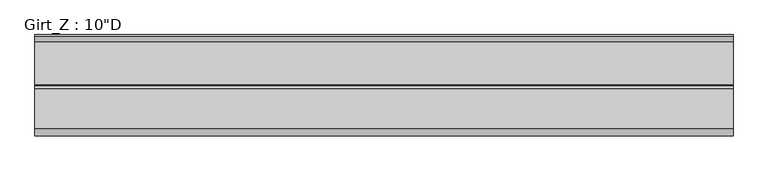
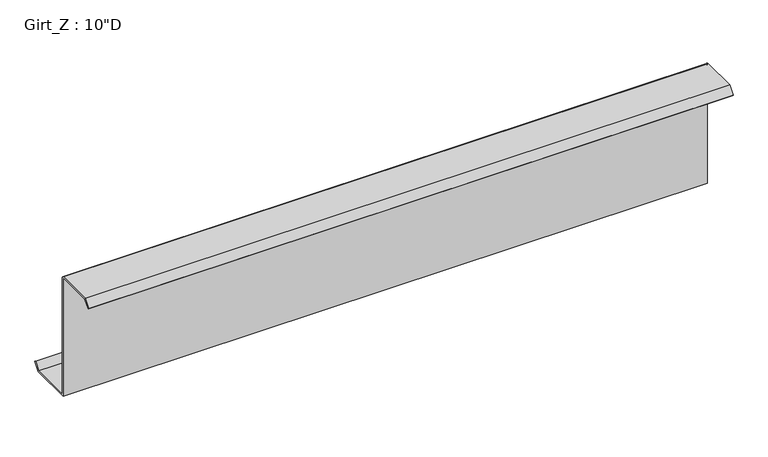
"""IFC4 building model written with IfcOpenShell, lengths in millimetres: beam geometry."""

from ifc_helpers import new_model, si_unit, point, frame, frame_2d, origin, place, context, project, spatial, polyline, circle_curve, trimmed, segment, composite_curve, outline, extrude, source, transform, mapped, element, save


def beam_41f086bf(model_context):
    return source(origin(), model_context, "Body", "SweptSolid", [
        extrude(outline(composite_curve([segment(polyline([(-77.9859375, 127.0), (-3.3734375, 127.0)]), True, "CONTINUOUS"), segment(trimmed(circle_curve(frame_2d((-3.3734375, 122.2375)), 4.7625), [point((-3.3734375, 127.0))], [point((1.3890625, 122.2375))], False, "CARTESIAN"), True, "CONTINUOUS"), segment(polyline([(1.3890625, 122.2375), (1.3890625, -122.2389339)]), True, "CONTINUOUS"), segment(trimmed(circle_curve(frame_2d((3.3748024, -122.2389339)), 1.9857399), [point((1.3890625, -122.2389339))], [point((3.2694106, -124.221875))], True, "CARTESIAN"), True, "CONTINUOUS"), segment(polyline([(3.2694106, -124.221875), (83.0404765, -124.221875), (94.4528742, -110.621109), (96.5810415, -112.4068534), (84.3359375, -127.0), (-1.3890625, -127.0), (-1.3890625, 122.2381931)]), True, "CONTINUOUS"), segment(trimmed(circle_curve(frame_2d((-3.3741066, 122.2381931)), 1.9850441), [point((-1.3890625, 122.2381931))], [point((-3.3005807, 124.221875))], True, "CARTESIAN"), True, "CONTINUOUS"), segment(polyline([(-3.3005807, 124.221875), (-76.6904765, 124.221875), (-88.1028742, 110.621109), (-90.2310415, 112.4068534), (-77.9859375, 127.0)]), True, "CONTINUOUS")], self_intersect=False)), frame((-689.0766, 0.0, 0.0), z_axis=(1.0, 0.0, 0.0), x_axis=(0.0, 1.0, 0.0)), (0.0, 0.0, 1.0), 1288.669),
    ])


if __name__ == "__main__":
    model = new_model("IFC4")
    model_context = context("Model", 3, world=origin())
    ifc_project = project(units=[si_unit("LENGTHUNIT", "METRE", prefix="MILLI")], contexts=[model_context])
    site = spatial("IfcSite", under=ifc_project)
    building = spatial("IfcBuilding", under=site)
    placement = place(None, origin())
    beam_shape = beam_41f086bf(model_context)
    element("IfcBeam", 1, ObjectType="Girt_Z : 10\"D", at=placement, inside=building, context=model_context, shape_type="MappedRepresentation", body=[
        mapped(beam_shape, transform((0.0, 0.0, 0.0), x_axis=(1.0, 0.0, 0.0), y_axis=(0.0, 1.0, 0.0), z_axis=(0.0, 0.0, 1.0))),
    ])
    save(model, "model.ifc")

# Revit data of these elements
# Type "Girt_Z : 10\"D"
#   half leg = 0' - 1 11/16"
#   Web_Thickness = 0' - 0 7/64"
#   Length [instance default] = 10' - 0"
#   Leg_2 = 0' - 3 3/8"
#   Leg_1 = 0' - 3 1/8"
#   Height = 0' - 10"
#   Structural Material [instance default] = none
# Element 1 (IfcBeam, "Girt_Z : 10\"D")
#   Structural Material = STRUCTURAL STEEL - SEE STRUCT. DWGS
#   Materials on its faces: "STRUCTURAL STEEL - SEE STRUCT. DWGS"
# Materials
#   "STRUCTURAL STEEL - SEE STRUCT. DWGS": class "Metal", colour RGB 137 146 153, transparency 0, Description = "Steel, mill finish", Cost = 0
